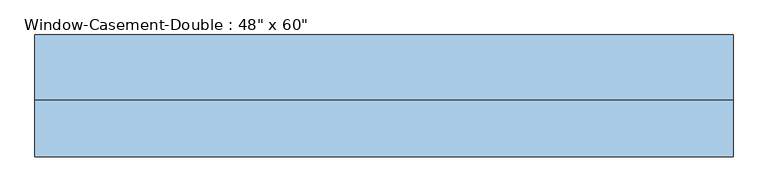
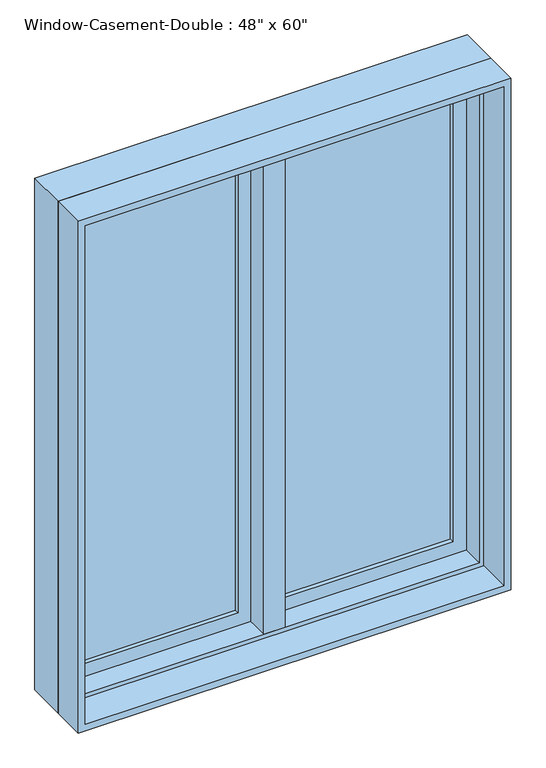
"""IFC4 building model written with IfcOpenShell, lengths in millimetres: window geometry."""

from ifc_helpers import new_model, si_unit, frame, origin, place, context, project, spatial, polyline, outline, extrude, faceted_brep, source, transform, mapped, element, save


def window_d7f95d13(model_context):
    return source(origin(), model_context, "Body", "SolidModel", [
        faceted_brep([(9.525, 115.8875, 2425.7), (-9.525, 115.8875, 2425.7), (-9.525, 65.0875, 2425.7), (9.525, 65.0875, 2425.7), (9.525, 115.8875, 927.1), (9.525, 65.0875, 927.1), (-9.525, 65.0875, 927.1), (-9.525, 115.8875, 927.1), (-9.525, 65.0875, 946.15), (-9.525, 65.0875, 2406.65), (-30.1625, 65.0875, 946.15), (-30.1625, 65.0875, 2406.65), (-30.1625, 1.5875, 946.15), (-30.1625, 1.5875, 2406.65), (30.1625, 1.5875, 946.15), (30.1625, 1.5875, 2406.65), (30.1625, 65.0875, 946.15), (30.1625, 65.0875, 2406.65), (9.525, 65.0875, 946.15), (9.525, 65.0875, 2406.65)], [[[0, 1, 2, 3]], [[4, 5, 6, 7]], [[1, 0, 4, 7]], [[2, 1, 7, 6, 8, 9]], [[9, 8, 10, 11]], [[11, 10, 12, 13]], [[13, 12, 14, 15]], [[15, 14, 16, 17]], [[17, 16, 18, 19]], [[0, 3, 19, 18, 5, 4]], [[18, 8, 6, 5]], [[9, 19, 3, 2]], [[8, 18, 16, 14, 12, 10]], [[19, 9, 11, 13, 15, 17]]]),
        extrude(outline(polyline([(-66.675, 96.8375), (-66.675, 90.4875), (-539.75, 90.4875), (-539.75, 96.8375), (-66.675, 96.8375)])), frame((0.0, 0.0, 984.25), z_axis=(0.0, 0.0, 1.0), x_axis=(1.0, 0.0, 0.0)), (0.0, 0.0, 1.0), 1384.3),
        extrude(outline(polyline([(-539.75, 77.7875), (-539.75, 84.1375), (-66.675, 84.1375), (-66.675, 77.7875), (-539.75, 77.7875)])), frame((0.0, 0.0, 984.25), z_axis=(0.0, 0.0, 1.0), x_axis=(1.0, 0.0, 0.0)), (0.0, 0.0, 1.0), 1384.3),
        extrude(outline(polyline([(539.75, 96.8375), (539.75, 90.4875), (66.675, 90.4875), (66.675, 96.8375), (539.75, 96.8375)])), frame((0.0, 0.0, 984.25), z_axis=(0.0, 0.0, 1.0), x_axis=(1.0, 0.0, 0.0)), (0.0, 0.0, 1.0), 1384.3),
        extrude(outline(polyline([(66.675, 77.7875), (66.675, 84.1375), (539.75, 84.1375), (539.75, 77.7875), (66.675, 77.7875)])), frame((0.0, 0.0, 984.25), z_axis=(0.0, 0.0, 1.0), x_axis=(1.0, 0.0, 0.0)), (0.0, 0.0, 1.0), 1384.3),
        extrude(outline(polyline([(2425.7, -596.9), (927.1, -596.9), (927.1, -9.525), (2425.7, -9.525), (2425.7, -596.9)]), holes=[polyline([(2368.55, -66.675), (984.25, -66.675), (984.25, -539.75), (2368.55, -539.75), (2368.55, -66.675)])]), frame((0.0, 65.0875, 0.0), z_axis=(0.0, 1.0, 0.0), x_axis=(0.0, 0.0, 1.0)), (0.0, 0.0, 1.0), 44.45),
        extrude(outline(polyline([(927.1, 596.9), (2425.7, 596.9), (2425.7, 9.525), (927.1, 9.525), (927.1, 596.9)]), holes=[polyline([(984.25, 66.675), (2368.55, 66.675), (2368.55, 539.75), (984.25, 539.75), (984.25, 66.675)])]), frame((0.0, 65.0875, 0.0), z_axis=(0.0, 1.0, 0.0), x_axis=(0.0, 0.0, 1.0)), (0.0, 0.0, 1.0), 44.45),
        extrude(outline(polyline([(2438.4, -609.6), (914.4, -609.6), (914.4, 609.6), (2438.4, 609.6), (2438.4, -609.6)]), holes=[polyline([(2419.35, 590.55), (933.45, 590.55), (933.45, -590.55), (2419.35, -590.55), (2419.35, 590.55)])]), frame((0.0, -96.8375, 0.0), z_axis=(0.0, 1.0, 0.0), x_axis=(0.0, 0.0, 1.0)), (0.0, 0.0, 1.0), 98.425),
        faceted_brep([(577.85, 65.0875, 2406.65), (577.85, 1.5875, 2406.65), (-577.85, 1.5875, 2406.65), (-577.85, 65.0875, 2406.65), (596.9, 115.8875, 2425.7), (596.9, 65.0875, 2425.7), (-596.9, 65.0875, 2425.7), (-596.9, 115.8875, 2425.7), (609.6, 1.5875, 2438.4), (609.6, 115.8875, 2438.4), (-609.6, 115.8875, 2438.4), (-609.6, 1.5875, 2438.4), (-577.85, 1.5875, 946.15), (-577.85, 65.0875, 946.15), (-596.9, 65.0875, 927.1), (-596.9, 115.8875, 927.1), (-609.6, 115.8875, 914.4), (-609.6, 1.5875, 914.4), (577.85, 1.5875, 946.15), (577.85, 65.0875, 946.15), (596.9, 65.0875, 927.1), (596.9, 115.8875, 927.1), (609.6, 115.8875, 914.4), (609.6, 1.5875, 914.4)], [[[0, 1, 2, 3]], [[4, 5, 6, 7]], [[8, 9, 10, 11]], [[3, 2, 12, 13]], [[7, 6, 14, 15]], [[11, 10, 16, 17]], [[13, 12, 18, 19]], [[15, 14, 20, 21]], [[17, 16, 22, 23]], [[11, 17, 23, 8], [1, 18, 12, 2]], [[19, 18, 1, 0]], [[5, 20, 14, 6], [3, 13, 19, 0]], [[21, 20, 5, 4]], [[23, 22, 9, 8]], [[9, 22, 16, 10], [7, 15, 21, 4]]]),
    ])


if __name__ == "__main__":
    model = new_model("IFC4")
    model_context = context("Model", 3, world=origin())
    ifc_project = project(units=[si_unit("LENGTHUNIT", "METRE", prefix="MILLI")], contexts=[model_context])
    site = spatial("IfcSite", under=ifc_project)
    building = spatial("IfcBuilding", under=site)
    placement = place(None, origin())
    window_shape = window_d7f95d13(model_context)
    element("IfcWindow", 1, ObjectType="Window-Casement-Double : 48\" x 60\"", at=placement, inside=building, context=model_context, shape_type="MappedRepresentation", body=[
        mapped(window_shape, transform((0.0, 0.0, 0.0), x_axis=(1.0, 0.0, 0.0), y_axis=(0.0, 1.0, 0.0), z_axis=(0.0, 0.0, 1.0))),
    ])
    save(model, "model.ifc")

# Revit data of these elements
# Type "Window-Casement-Double : 48\" x 60\""
#   Type Mark = "61"
#   Fire Rating = "0.5h"
#   Assembly Code = "B2020100"
#   Analytic Construction = "Double glazing - domestic"
#   Frame Extension [instance default] = 0' - 0 1/4"
#   Window Inset [instance default] = 0' - 0"
#   Wall Thickness [instance default] = 0' - 6"
#   Interior Wall Closure [instance default] = 0' - 2 1/4"
#   Half Width = 2' - 0"
#   Visual Light Transmittance = 0.81
#   Thermal Resistance (R) = 1.8146 (h·ft²·°F)/BTU
#   Solar Heat Gain Coefficient = 0.76
#   Rough Width = 4' - 0 1/2"
#   Rough Height = 5' - 0 1/2"
#   Height = 5' - 0"
#   Heat Transfer Coefficient (U) = 0.5511 BTU/(h·ft²·°F)
#   Exterior Wall Closure [instance default] = 0' - 1 1/4"
#   Extension Jamb [instance default] = 0' - 2 1/4"
#   Default Sill Height = 3' - 0"
#   Width = 4' - 0"
#   Define Thermal Properties by = 0
#   Muntin Visibility = yes
#   Interior Trim Visibility [instance default] = yes
#   Exterior Trim Visibility [instance default] = yes
#   Extension Jamb Visibility [instance default] = yes
#   Interior Trim Material = Wood - Stained
#   Muntin Pattern = Muntin Pattern_2x2 : Muntin Pattern_2x2
#   Interior Trim = Trim-Window-Interior-Flat : Picture Frame
#   Interior Frame Material = Wood - Stained
#   Glass Panel Material = Glass
#   Exterior Trim Material = Clad - White
#   Exterior Trim = Trim-Window-Exterior-Flat : with Sill
#   Exterior Frame Material = Clad - White
#   Wall Closure = (empty or 0)
# Element 1 (IfcWindow, "Window-Casement-Double : 48\" x 60\"")
#   Wall Thickness = 0' - 7 5/8"
#   Extension Jamb = 0' - 3 7/8"
#   Materials on its faces: "Wood - Stained", "Glass", "Clad - White"
# Materials
#   "Wood - Stained": class "Wood", colour RGB 224 178 126, transparency 0, Cost = 0
#   "Glass": class "Glass", colour RGB 236 240 239, transparency 0.5, Description = "Soda Lime Glass", Cost = 0
#   "Clad - White": class "Wood", colour RGB 216 216 204, transparency 0, Cost = 0
